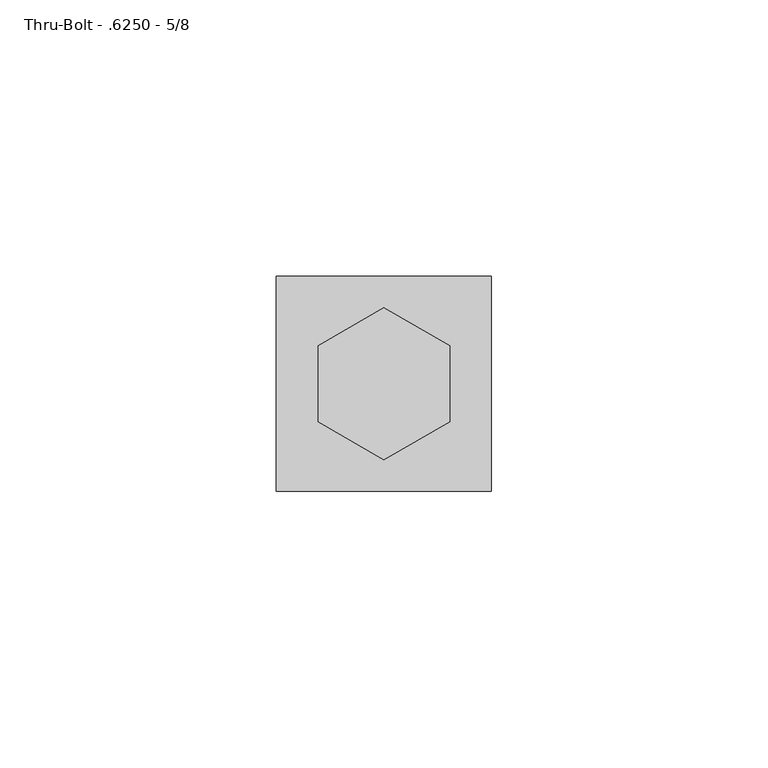
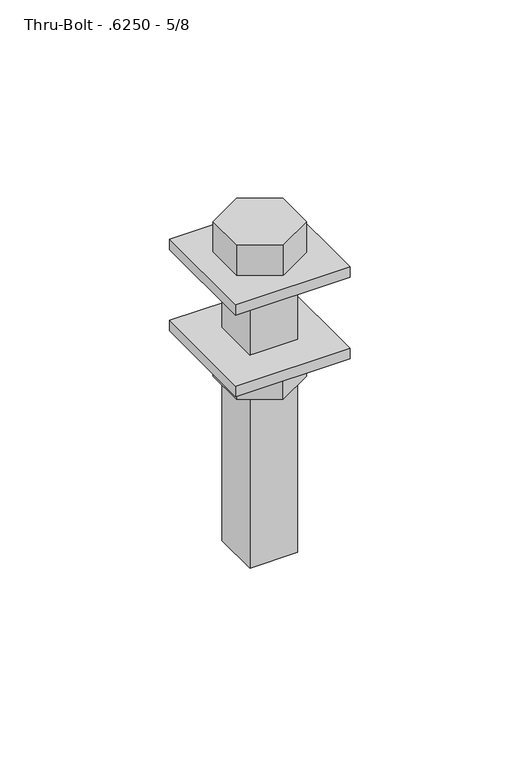
"""IFC4 building model written with IfcOpenShell, lengths in millimetres: fastener geometry, 060523 - W_P_C - Fastenings - Generic - SQUARE : Thru-Bolt - .6250 - 5/8."""

from ifc_helpers import new_model, si_unit, frame, origin, origin_with_axes, place, context, project, spatial, polyline, outline, extrude, source, transform, mapped, element, save


def thru_bolt_6250_5_8_f1e17e93(model_context):
    return source(origin(), model_context, "Body", "SweptSolid", [
        extrude(outline(polyline([(-19.446875, -19.446875), (-19.446875, 19.446875), (19.446875, 19.446875), (19.446875, -19.446875), (-19.446875, -19.446875)])), origin_with_axes(), (0.0, 0.0, 1.0), 3.7703125),
        extrude(outline(polyline([(-19.446875, -19.446875), (-19.446875, 19.446875), (19.446875, 19.446875), (19.446875, -19.446875), (-19.446875, -19.446875)])), frame((0.0, 0.0, -29.1703125), z_axis=(0.0, 0.0, 1.0), x_axis=(1.0, 0.0, 0.0)), (0.0, 0.0, 1.0), 3.7703125),
        extrude(outline(polyline([(-11.90625, -6.8740766), (-11.90625, 6.8740766), (0.0, 13.7481533), (11.90625, 6.8740766), (11.90625, -6.8740766), (0.0, -13.7481533), (-11.90625, -6.8740766)])), frame((0.0, 0.0, -40.48125), z_axis=(0.0, 0.0, 1.0), x_axis=(1.0, 0.0, 0.0)), (0.0, 0.0, 1.0), 11.3109375),
        extrude(outline(polyline([(-11.90625, 6.8740766), (0.0, 13.7481533), (11.90625, 6.8740766), (11.90625, -6.8740766), (0.0, -13.7481533), (-11.90625, -6.8740766), (-11.90625, 6.8740766)])), frame((0.0, 0.0, 3.7703125), z_axis=(0.0, 0.0, 1.0), x_axis=(1.0, 0.0, 0.0)), (0.0, 0.0, 1.0), 11.3109375),
        extrude(outline(polyline([(-8.1359375, 8.1359375), (8.1359375, 8.1359375), (8.1359375, -8.1359375), (-8.1359375, -8.1359375), (-8.1359375, 8.1359375)])), frame((0.0, 0.0, -101.6), z_axis=(0.0, 0.0, 1.0), x_axis=(1.0, 0.0, 0.0)), (0.0, 0.0, 1.0), 105.3703125),
    ])


if __name__ == "__main__":
    model = new_model("IFC4")
    model_context = context("Model", 3, world=origin())
    ifc_project = project(units=[si_unit("LENGTHUNIT", "METRE", prefix="MILLI")], contexts=[model_context])
    site = spatial("IfcSite", under=ifc_project)
    building = spatial("IfcBuilding", under=site)
    placement = place(None, origin())
    thru_bolt_6250_5_8_shape = thru_bolt_6250_5_8_f1e17e93(model_context)
    element("IfcFastener", 1, ObjectType="060523 - W_P_C - Fastenings - Generic - SQUARE : Thru-Bolt - .6250 - 5/8", at=placement, inside=building, context=model_context, shape_type="MappedRepresentation", body=[
        mapped(thru_bolt_6250_5_8_shape, transform((0.0, 0.0, 0.0), x_axis=(1.0, 0.0, 0.0), y_axis=(0.0, 1.0, 0.0), z_axis=(0.0, 0.0, 1.0))),
    ])
    save(model, "model.ifc")

# Revit data of these elements
# Type "060523 - W_P_C - Fastenings - Generic - SQUARE : Thru-Bolt - .6250 - 5/8"
#   Washer_Thickness = 0' - 0 19/128"
#   Washer Radius = 0' - 0 49/64"
#   Washer Offset - Head = 0' - 0 19/128"
#   Washer Offset = 0' - 0 19/128"
#   Thickness_of_Substrate [instance default] = 0' - 1"
#   Side = 0' - 0.54199"
#   Radius = 0' - 0 41/128"
#   Length [instance default] = 0' - 4"
#   Head Size = 0' - 0 15/16"
#   Head Radius = 0' - 0 15/32"
#   Head Height = 0' - 0 57/128"
#   Double Diameter = 0' - 1 9/32"
#   Diameter = 0' - 0 41/64"
#   Default Elevation = 4' - 0"
#   Washer_Nut_Visibility = yes
#   Washer_Head_Visibility = yes
#   Round_Head_Visibility = no
#   Point Visibility = no
#   Nut_Visibility = yes
#   Hex_Head_Visiblilty = yes
#   Washer Material = none
#   Bolt Material (Size) = AT SILL - FASTENER AT 24" O.C.
# Element 1 (IfcFastener, "060523 - W_P_C - Fastenings - Generic - SQUARE : Thru-Bolt - .6250 - 5/8")
#   Materials on its faces: "AT SILL - FASTENER AT 24\" O.C."
# Materials
#   "AT SILL - FASTENER AT 24\" O.C.": class "Generic", colour RGB 120 120 120, transparency 0, Cost = 0
